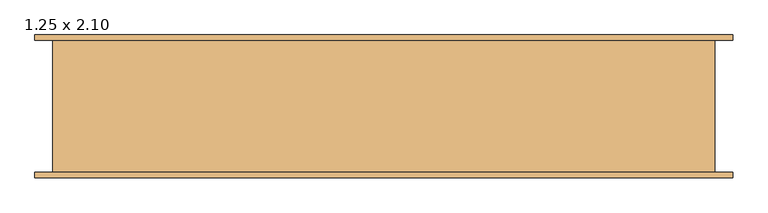
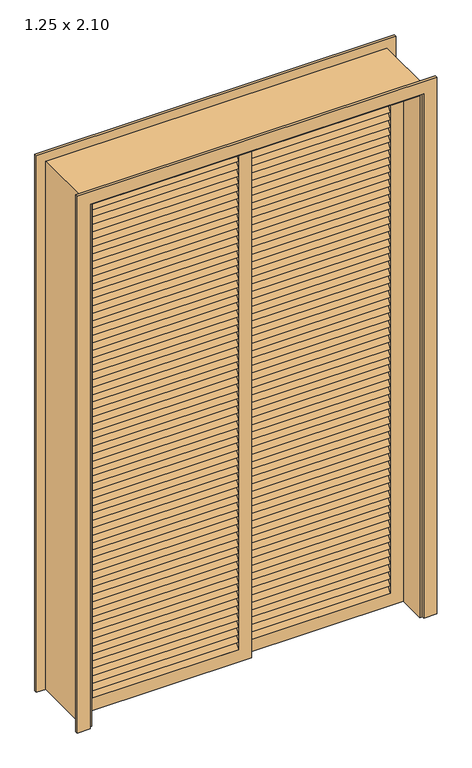
"""IFC4 building model written with IfcOpenShell, lengths in millimetres: door geometry, .CC_ND 300_PORTA DE CORRER_3 FOLHAS_VENEZIANA_VIDRO_COM EXTENSÃO : 1.25 x 2.10."""

from ifc_helpers import new_model, si_unit, frame, origin, place, context, project, spatial, polyline, outline, extrude, source, transform, mapped, element, save


def door_1_25_x_2_10_052434fb(model_context):
    return source(origin(), model_context, "Body", "SweptSolid", [
        extrude(outline(polyline([(575.0, 26.0), (20.0, 26.0), (20.0, 34.0), (575.0, 34.0), (575.0, 26.0)])), frame((0.0, 0.0, 50.0), z_axis=(0.0, 0.0, 1.0), x_axis=(1.0, 0.0, 0.0)), (0.0, 0.0, 1.0), 2000.0),
        extrude(outline(polyline([(2100.0, 625.0), (2100.0, -30.0), (0.0, -30.0), (0.0, 625.0), (2100.0, 625.0)]), holes=[polyline([(2050.0, 575.0), (50.0, 575.0), (50.0, 20.0), (2050.0, 20.0), (2050.0, 575.0)])]), frame((0.0, 15.0, 0.0), z_axis=(0.0, 1.0, 0.0), x_axis=(0.0, 0.0, 1.0)), (0.0, 0.0, 1.0), 30.0),
        extrude(outline(polyline([(-40.0, 1985.2272727), (-45.0, 1985.2272727), (-20.0, 2020.2272727), (-15.0, 2020.2272727), (-40.0, 1985.2272727)])), frame((-575.0, 0.0, 0.0), z_axis=(1.0, 0.0, 0.0), x_axis=(0.0, 1.0, 0.0)), (0.0, 0.0, 1.0), 555.0),
        extrude(outline(polyline([(-40.0, 1955.4545455), (-45.0, 1955.4545455), (-20.0, 1990.4545455), (-15.0, 1990.4545455), (-40.0, 1955.4545455)])), frame((-575.0, 0.0, 0.0), z_axis=(1.0, 0.0, 0.0), x_axis=(0.0, 1.0, 0.0)), (0.0, 0.0, 1.0), 555.0),
        extrude(outline(polyline([(-40.0, 1925.6818182), (-45.0, 1925.6818182), (-20.0, 1960.6818182), (-15.0, 1960.6818182), (-40.0, 1925.6818182)])), frame((-575.0, 0.0, 0.0), z_axis=(1.0, 0.0, 0.0), x_axis=(0.0, 1.0, 0.0)), (0.0, 0.0, 1.0), 555.0),
        extrude(outline(polyline([(-40.0, 1895.9090909), (-45.0, 1895.9090909), (-20.0, 1930.9090909), (-15.0, 1930.9090909), (-40.0, 1895.9090909)])), frame((-575.0, 0.0, 0.0), z_axis=(1.0, 0.0, 0.0), x_axis=(0.0, 1.0, 0.0)), (0.0, 0.0, 1.0), 555.0),
        extrude(outline(polyline([(-40.0, 1866.1363636), (-45.0, 1866.1363636), (-20.0, 1901.1363636), (-15.0, 1901.1363636), (-40.0, 1866.1363636)])), frame((-575.0, 0.0, 0.0), z_axis=(1.0, 0.0, 0.0), x_axis=(0.0, 1.0, 0.0)), (0.0, 0.0, 1.0), 555.0),
        extrude(outline(polyline([(-40.0, 1836.3636364), (-45.0, 1836.3636364), (-20.0, 1871.3636364), (-15.0, 1871.3636364), (-40.0, 1836.3636364)])), frame((-575.0, 0.0, 0.0), z_axis=(1.0, 0.0, 0.0), x_axis=(0.0, 1.0, 0.0)), (0.0, 0.0, 1.0), 555.0),
        extrude(outline(polyline([(-40.0, 1806.5909091), (-45.0, 1806.5909091), (-20.0, 1841.5909091), (-15.0, 1841.5909091), (-40.0, 1806.5909091)])), frame((-575.0, 0.0, 0.0), z_axis=(1.0, 0.0, 0.0), x_axis=(0.0, 1.0, 0.0)), (0.0, 0.0, 1.0), 555.0),
        extrude(outline(polyline([(-40.0, 1776.8181818), (-45.0, 1776.8181818), (-20.0, 1811.8181818), (-15.0, 1811.8181818), (-40.0, 1776.8181818)])), frame((-575.0, 0.0, 0.0), z_axis=(1.0, 0.0, 0.0), x_axis=(0.0, 1.0, 0.0)), (0.0, 0.0, 1.0), 555.0),
        extrude(outline(polyline([(-40.0, 1747.0454545), (-45.0, 1747.0454545), (-20.0, 1782.0454545), (-15.0, 1782.0454545), (-40.0, 1747.0454545)])), frame((-575.0, 0.0, 0.0), z_axis=(1.0, 0.0, 0.0), x_axis=(0.0, 1.0, 0.0)), (0.0, 0.0, 1.0), 555.0),
        extrude(outline(polyline([(-40.0, 1717.2727273), (-45.0, 1717.2727273), (-20.0, 1752.2727273), (-15.0, 1752.2727273), (-40.0, 1717.2727273)])), frame((-575.0, 0.0, 0.0), z_axis=(1.0, 0.0, 0.0), x_axis=(0.0, 1.0, 0.0)), (0.0, 0.0, 1.0), 555.0),
        extrude(outline(polyline([(-40.0, 1687.5), (-45.0, 1687.5), (-20.0, 1722.5), (-15.0, 1722.5), (-40.0, 1687.5)])), frame((-575.0, 0.0, 0.0), z_axis=(1.0, 0.0, 0.0), x_axis=(0.0, 1.0, 0.0)), (0.0, 0.0, 1.0), 555.0),
        extrude(outline(polyline([(-40.0, 1657.7272727), (-45.0, 1657.7272727), (-20.0, 1692.7272727), (-15.0, 1692.7272727), (-40.0, 1657.7272727)])), frame((-575.0, 0.0, 0.0), z_axis=(1.0, 0.0, 0.0), x_axis=(0.0, 1.0, 0.0)), (0.0, 0.0, 1.0), 555.0),
        extrude(outline(polyline([(-40.0, 1627.9545455), (-45.0, 1627.9545455), (-20.0, 1662.9545455), (-15.0, 1662.9545455), (-40.0, 1627.9545455)])), frame((-575.0, 0.0, 0.0), z_axis=(1.0, 0.0, 0.0), x_axis=(0.0, 1.0, 0.0)), (0.0, 0.0, 1.0), 555.0),
        extrude(outline(polyline([(-40.0, 1598.1818182), (-45.0, 1598.1818182), (-20.0, 1633.1818182), (-15.0, 1633.1818182), (-40.0, 1598.1818182)])), frame((-575.0, 0.0, 0.0), z_axis=(1.0, 0.0, 0.0), x_axis=(0.0, 1.0, 0.0)), (0.0, 0.0, 1.0), 555.0),
        extrude(outline(polyline([(-40.0, 1568.4090909), (-45.0, 1568.4090909), (-20.0, 1603.4090909), (-15.0, 1603.4090909), (-40.0, 1568.4090909)])), frame((-575.0, 0.0, 0.0), z_axis=(1.0, 0.0, 0.0), x_axis=(0.0, 1.0, 0.0)), (0.0, 0.0, 1.0), 555.0),
        extrude(outline(polyline([(-40.0, 1538.6363636), (-45.0, 1538.6363636), (-20.0, 1573.6363636), (-15.0, 1573.6363636), (-40.0, 1538.6363636)])), frame((-575.0, 0.0, 0.0), z_axis=(1.0, 0.0, 0.0), x_axis=(0.0, 1.0, 0.0)), (0.0, 0.0, 1.0), 555.0),
        extrude(outline(polyline([(-40.0, 1508.8636364), (-45.0, 1508.8636364), (-20.0, 1543.8636364), (-15.0, 1543.8636364), (-40.0, 1508.8636364)])), frame((-575.0, 0.0, 0.0), z_axis=(1.0, 0.0, 0.0), x_axis=(0.0, 1.0, 0.0)), (0.0, 0.0, 1.0), 555.0),
        extrude(outline(polyline([(-40.0, 1479.0909091), (-45.0, 1479.0909091), (-20.0, 1514.0909091), (-15.0, 1514.0909091), (-40.0, 1479.0909091)])), frame((-575.0, 0.0, 0.0), z_axis=(1.0, 0.0, 0.0), x_axis=(0.0, 1.0, 0.0)), (0.0, 0.0, 1.0), 555.0),
        extrude(outline(polyline([(-40.0, 1449.3181818), (-45.0, 1449.3181818), (-20.0, 1484.3181818), (-15.0, 1484.3181818), (-40.0, 1449.3181818)])), frame((-575.0, 0.0, 0.0), z_axis=(1.0, 0.0, 0.0), x_axis=(0.0, 1.0, 0.0)), (0.0, 0.0, 1.0), 555.0),
        extrude(outline(polyline([(-40.0, 1419.5454545), (-45.0, 1419.5454545), (-20.0, 1454.5454545), (-15.0, 1454.5454545), (-40.0, 1419.5454545)])), frame((-575.0, 0.0, 0.0), z_axis=(1.0, 0.0, 0.0), x_axis=(0.0, 1.0, 0.0)), (0.0, 0.0, 1.0), 555.0),
        extrude(outline(polyline([(-40.0, 1389.7727273), (-45.0, 1389.7727273), (-20.0, 1424.7727273), (-15.0, 1424.7727273), (-40.0, 1389.7727273)])), frame((-575.0, 0.0, 0.0), z_axis=(1.0, 0.0, 0.0), x_axis=(0.0, 1.0, 0.0)), (0.0, 0.0, 1.0), 555.0),
        extrude(outline(polyline([(-40.0, 1360.0), (-45.0, 1360.0), (-20.0, 1395.0), (-15.0, 1395.0), (-40.0, 1360.0)])), frame((-575.0, 0.0, 0.0), z_axis=(1.0, 0.0, 0.0), x_axis=(0.0, 1.0, 0.0)), (0.0, 0.0, 1.0), 555.0),
        extrude(outline(polyline([(-40.0, 1330.2272727), (-45.0, 1330.2272727), (-20.0, 1365.2272727), (-15.0, 1365.2272727), (-40.0, 1330.2272727)])), frame((-575.0, 0.0, 0.0), z_axis=(1.0, 0.0, 0.0), x_axis=(0.0, 1.0, 0.0)), (0.0, 0.0, 1.0), 555.0),
        extrude(outline(polyline([(-40.0, 1300.4545455), (-45.0, 1300.4545455), (-20.0, 1335.4545455), (-15.0, 1335.4545455), (-40.0, 1300.4545455)])), frame((-575.0, 0.0, 0.0), z_axis=(1.0, 0.0, 0.0), x_axis=(0.0, 1.0, 0.0)), (0.0, 0.0, 1.0), 555.0),
        extrude(outline(polyline([(-40.0, 1270.6818182), (-45.0, 1270.6818182), (-20.0, 1305.6818182), (-15.0, 1305.6818182), (-40.0, 1270.6818182)])), frame((-575.0, 0.0, 0.0), z_axis=(1.0, 0.0, 0.0), x_axis=(0.0, 1.0, 0.0)), (0.0, 0.0, 1.0), 555.0),
        extrude(outline(polyline([(-40.0, 1240.9090909), (-45.0, 1240.9090909), (-20.0, 1275.9090909), (-15.0, 1275.9090909), (-40.0, 1240.9090909)])), frame((-575.0, 0.0, 0.0), z_axis=(1.0, 0.0, 0.0), x_axis=(0.0, 1.0, 0.0)), (0.0, 0.0, 1.0), 555.0),
        extrude(outline(polyline([(-40.0, 1211.1363636), (-45.0, 1211.1363636), (-20.0, 1246.1363636), (-15.0, 1246.1363636), (-40.0, 1211.1363636)])), frame((-575.0, 0.0, 0.0), z_axis=(1.0, 0.0, 0.0), x_axis=(0.0, 1.0, 0.0)), (0.0, 0.0, 1.0), 555.0),
        extrude(outline(polyline([(-40.0, 1181.3636364), (-45.0, 1181.3636364), (-20.0, 1216.3636364), (-15.0, 1216.3636364), (-40.0, 1181.3636364)])), frame((-575.0, 0.0, 0.0), z_axis=(1.0, 0.0, 0.0), x_axis=(0.0, 1.0, 0.0)), (0.0, 0.0, 1.0), 555.0),
        extrude(outline(polyline([(-40.0, 1151.5909091), (-45.0, 1151.5909091), (-20.0, 1186.5909091), (-15.0, 1186.5909091), (-40.0, 1151.5909091)])), frame((-575.0, 0.0, 0.0), z_axis=(1.0, 0.0, 0.0), x_axis=(0.0, 1.0, 0.0)), (0.0, 0.0, 1.0), 555.0),
        extrude(outline(polyline([(-40.0, 1121.8181818), (-45.0, 1121.8181818), (-20.0, 1156.8181818), (-15.0, 1156.8181818), (-40.0, 1121.8181818)])), frame((-575.0, 0.0, 0.0), z_axis=(1.0, 0.0, 0.0), x_axis=(0.0, 1.0, 0.0)), (0.0, 0.0, 1.0), 555.0),
        extrude(outline(polyline([(-40.0, 1092.0454545), (-45.0, 1092.0454545), (-20.0, 1127.0454545), (-15.0, 1127.0454545), (-40.0, 1092.0454545)])), frame((-575.0, 0.0, 0.0), z_axis=(1.0, 0.0, 0.0), x_axis=(0.0, 1.0, 0.0)), (0.0, 0.0, 1.0), 555.0),
        extrude(outline(polyline([(-40.0, 1062.2727273), (-45.0, 1062.2727273), (-20.0, 1097.2727273), (-15.0, 1097.2727273), (-40.0, 1062.2727273)])), frame((-575.0, 0.0, 0.0), z_axis=(1.0, 0.0, 0.0), x_axis=(0.0, 1.0, 0.0)), (0.0, 0.0, 1.0), 555.0),
        extrude(outline(polyline([(-40.0, 1032.5), (-45.0, 1032.5), (-20.0, 1067.5), (-15.0, 1067.5), (-40.0, 1032.5)])), frame((-575.0, 0.0, 0.0), z_axis=(1.0, 0.0, 0.0), x_axis=(0.0, 1.0, 0.0)), (0.0, 0.0, 1.0), 555.0),
        extrude(outline(polyline([(-40.0, 1002.7272727), (-45.0, 1002.7272727), (-20.0, 1037.7272727), (-15.0, 1037.7272727), (-40.0, 1002.7272727)])), frame((-575.0, 0.0, 0.0), z_axis=(1.0, 0.0, 0.0), x_axis=(0.0, 1.0, 0.0)), (0.0, 0.0, 1.0), 555.0),
        extrude(outline(polyline([(-40.0, 972.9545455), (-45.0, 972.9545455), (-20.0, 1007.9545455), (-15.0, 1007.9545455), (-40.0, 972.9545455)])), frame((-575.0, 0.0, 0.0), z_axis=(1.0, 0.0, 0.0), x_axis=(0.0, 1.0, 0.0)), (0.0, 0.0, 1.0), 555.0),
        extrude(outline(polyline([(-40.0, 943.1818182), (-45.0, 943.1818182), (-20.0, 978.1818182), (-15.0, 978.1818182), (-40.0, 943.1818182)])), frame((-575.0, 0.0, 0.0), z_axis=(1.0, 0.0, 0.0), x_axis=(0.0, 1.0, 0.0)), (0.0, 0.0, 1.0), 555.0),
        extrude(outline(polyline([(-40.0, 913.4090909), (-45.0, 913.4090909), (-20.0, 948.4090909), (-15.0, 948.4090909), (-40.0, 913.4090909)])), frame((-575.0, 0.0, 0.0), z_axis=(1.0, 0.0, 0.0), x_axis=(0.0, 1.0, 0.0)), (0.0, 0.0, 1.0), 555.0),
        extrude(outline(polyline([(-40.0, 883.6363636), (-45.0, 883.6363636), (-20.0, 918.6363636), (-15.0, 918.6363636), (-40.0, 883.6363636)])), frame((-575.0, 0.0, 0.0), z_axis=(1.0, 0.0, 0.0), x_axis=(0.0, 1.0, 0.0)), (0.0, 0.0, 1.0), 555.0),
        extrude(outline(polyline([(-40.0, 853.8636364), (-45.0, 853.8636364), (-20.0, 888.8636364), (-15.0, 888.8636364), (-40.0, 853.8636364)])), frame((-575.0, 0.0, 0.0), z_axis=(1.0, 0.0, 0.0), x_axis=(0.0, 1.0, 0.0)), (0.0, 0.0, 1.0), 555.0),
        extrude(outline(polyline([(-40.0, 824.0909091), (-45.0, 824.0909091), (-20.0, 859.0909091), (-15.0, 859.0909091), (-40.0, 824.0909091)])), frame((-575.0, 0.0, 0.0), z_axis=(1.0, 0.0, 0.0), x_axis=(0.0, 1.0, 0.0)), (0.0, 0.0, 1.0), 555.0),
        extrude(outline(polyline([(-40.0, 794.3181818), (-45.0, 794.3181818), (-20.0, 829.3181818), (-15.0, 829.3181818), (-40.0, 794.3181818)])), frame((-575.0, 0.0, 0.0), z_axis=(1.0, 0.0, 0.0), x_axis=(0.0, 1.0, 0.0)), (0.0, 0.0, 1.0), 555.0),
        extrude(outline(polyline([(-40.0, 764.5454545), (-45.0, 764.5454545), (-20.0, 799.5454545), (-15.0, 799.5454545), (-40.0, 764.5454545)])), frame((-575.0, 0.0, 0.0), z_axis=(1.0, 0.0, 0.0), x_axis=(0.0, 1.0, 0.0)), (0.0, 0.0, 1.0), 555.0),
        extrude(outline(polyline([(-40.0, 734.7727273), (-45.0, 734.7727273), (-20.0, 769.7727273), (-15.0, 769.7727273), (-40.0, 734.7727273)])), frame((-575.0, 0.0, 0.0), z_axis=(1.0, 0.0, 0.0), x_axis=(0.0, 1.0, 0.0)), (0.0, 0.0, 1.0), 555.0),
        extrude(outline(polyline([(-40.0, 705.0), (-45.0, 705.0), (-20.0, 740.0), (-15.0, 740.0), (-40.0, 705.0)])), frame((-575.0, 0.0, 0.0), z_axis=(1.0, 0.0, 0.0), x_axis=(0.0, 1.0, 0.0)), (0.0, 0.0, 1.0), 555.0),
        extrude(outline(polyline([(-40.0, 675.2272727), (-45.0, 675.2272727), (-20.0, 710.2272727), (-15.0, 710.2272727), (-40.0, 675.2272727)])), frame((-575.0, 0.0, 0.0), z_axis=(1.0, 0.0, 0.0), x_axis=(0.0, 1.0, 0.0)), (0.0, 0.0, 1.0), 555.0),
        extrude(outline(polyline([(-40.0, 645.4545455), (-45.0, 645.4545455), (-20.0, 680.4545455), (-15.0, 680.4545455), (-40.0, 645.4545455)])), frame((-575.0, 0.0, 0.0), z_axis=(1.0, 0.0, 0.0), x_axis=(0.0, 1.0, 0.0)), (0.0, 0.0, 1.0), 555.0),
        extrude(outline(polyline([(-40.0, 615.6818182), (-45.0, 615.6818182), (-20.0, 650.6818182), (-15.0, 650.6818182), (-40.0, 615.6818182)])), frame((-575.0, 0.0, 0.0), z_axis=(1.0, 0.0, 0.0), x_axis=(0.0, 1.0, 0.0)), (0.0, 0.0, 1.0), 555.0),
        extrude(outline(polyline([(-40.0, 585.9090909), (-45.0, 585.9090909), (-20.0, 620.9090909), (-15.0, 620.9090909), (-40.0, 585.9090909)])), frame((-575.0, 0.0, 0.0), z_axis=(1.0, 0.0, 0.0), x_axis=(0.0, 1.0, 0.0)), (0.0, 0.0, 1.0), 555.0),
        extrude(outline(polyline([(-40.0, 556.1363636), (-45.0, 556.1363636), (-20.0, 591.1363636), (-15.0, 591.1363636), (-40.0, 556.1363636)])), frame((-575.0, 0.0, 0.0), z_axis=(1.0, 0.0, 0.0), x_axis=(0.0, 1.0, 0.0)), (0.0, 0.0, 1.0), 555.0),
        extrude(outline(polyline([(-40.0, 526.3636364), (-45.0, 526.3636364), (-20.0, 561.3636364), (-15.0, 561.3636364), (-40.0, 526.3636364)])), frame((-575.0, 0.0, 0.0), z_axis=(1.0, 0.0, 0.0), x_axis=(0.0, 1.0, 0.0)), (0.0, 0.0, 1.0), 555.0),
        extrude(outline(polyline([(-40.0, 496.5909091), (-45.0, 496.5909091), (-20.0, 531.5909091), (-15.0, 531.5909091), (-40.0, 496.5909091)])), frame((-575.0, 0.0, 0.0), z_axis=(1.0, 0.0, 0.0), x_axis=(0.0, 1.0, 0.0)), (0.0, 0.0, 1.0), 555.0),
        extrude(outline(polyline([(-40.0, 466.8181818), (-45.0, 466.8181818), (-20.0, 501.8181818), (-15.0, 501.8181818), (-40.0, 466.8181818)])), frame((-575.0, 0.0, 0.0), z_axis=(1.0, 0.0, 0.0), x_axis=(0.0, 1.0, 0.0)), (0.0, 0.0, 1.0), 555.0),
        extrude(outline(polyline([(-40.0, 437.0454545), (-45.0, 437.0454545), (-20.0, 472.0454545), (-15.0, 472.0454545), (-40.0, 437.0454545)])), frame((-575.0, 0.0, 0.0), z_axis=(1.0, 0.0, 0.0), x_axis=(0.0, 1.0, 0.0)), (0.0, 0.0, 1.0), 555.0),
        extrude(outline(polyline([(-40.0, 407.2727273), (-45.0, 407.2727273), (-20.0, 442.2727273), (-15.0, 442.2727273), (-40.0, 407.2727273)])), frame((-575.0, 0.0, 0.0), z_axis=(1.0, 0.0, 0.0), x_axis=(0.0, 1.0, 0.0)), (0.0, 0.0, 1.0), 555.0),
        extrude(outline(polyline([(-40.0, 377.5), (-45.0, 377.5), (-20.0, 412.5), (-15.0, 412.5), (-40.0, 377.5)])), frame((-575.0, 0.0, 0.0), z_axis=(1.0, 0.0, 0.0), x_axis=(0.0, 1.0, 0.0)), (0.0, 0.0, 1.0), 555.0),
        extrude(outline(polyline([(-40.0, 347.7272727), (-45.0, 347.7272727), (-20.0, 382.7272727), (-15.0, 382.7272727), (-40.0, 347.7272727)])), frame((-575.0, 0.0, 0.0), z_axis=(1.0, 0.0, 0.0), x_axis=(0.0, 1.0, 0.0)), (0.0, 0.0, 1.0), 555.0),
        extrude(outline(polyline([(-40.0, 317.9545455), (-45.0, 317.9545455), (-20.0, 352.9545455), (-15.0, 352.9545455), (-40.0, 317.9545455)])), frame((-575.0, 0.0, 0.0), z_axis=(1.0, 0.0, 0.0), x_axis=(0.0, 1.0, 0.0)), (0.0, 0.0, 1.0), 555.0),
        extrude(outline(polyline([(-40.0, 288.1818182), (-45.0, 288.1818182), (-20.0, 323.1818182), (-15.0, 323.1818182), (-40.0, 288.1818182)])), frame((-575.0, 0.0, 0.0), z_axis=(1.0, 0.0, 0.0), x_axis=(0.0, 1.0, 0.0)), (0.0, 0.0, 1.0), 555.0),
        extrude(outline(polyline([(-40.0, 258.4090909), (-45.0, 258.4090909), (-20.0, 293.4090909), (-15.0, 293.4090909), (-40.0, 258.4090909)])), frame((-575.0, 0.0, 0.0), z_axis=(1.0, 0.0, 0.0), x_axis=(0.0, 1.0, 0.0)), (0.0, 0.0, 1.0), 555.0),
        extrude(outline(polyline([(-40.0, 228.6363636), (-45.0, 228.6363636), (-20.0, 263.6363636), (-15.0, 263.6363636), (-40.0, 228.6363636)])), frame((-575.0, 0.0, 0.0), z_axis=(1.0, 0.0, 0.0), x_axis=(0.0, 1.0, 0.0)), (0.0, 0.0, 1.0), 555.0),
        extrude(outline(polyline([(-40.0, 198.8636364), (-45.0, 198.8636364), (-20.0, 233.8636364), (-15.0, 233.8636364), (-40.0, 198.8636364)])), frame((-575.0, 0.0, 0.0), z_axis=(1.0, 0.0, 0.0), x_axis=(0.0, 1.0, 0.0)), (0.0, 0.0, 1.0), 555.0),
        extrude(outline(polyline([(-40.0, 169.0909091), (-45.0, 169.0909091), (-20.0, 204.0909091), (-15.0, 204.0909091), (-40.0, 169.0909091)])), frame((-575.0, 0.0, 0.0), z_axis=(1.0, 0.0, 0.0), x_axis=(0.0, 1.0, 0.0)), (0.0, 0.0, 1.0), 555.0),
        extrude(outline(polyline([(-40.0, 139.3181818), (-45.0, 139.3181818), (-20.0, 174.3181818), (-15.0, 174.3181818), (-40.0, 139.3181818)])), frame((-575.0, 0.0, 0.0), z_axis=(1.0, 0.0, 0.0), x_axis=(0.0, 1.0, 0.0)), (0.0, 0.0, 1.0), 555.0),
        extrude(outline(polyline([(-40.0, 109.5454545), (-45.0, 109.5454545), (-20.0, 144.5454545), (-15.0, 144.5454545), (-40.0, 109.5454545)])), frame((-575.0, 0.0, 0.0), z_axis=(1.0, 0.0, 0.0), x_axis=(0.0, 1.0, 0.0)), (0.0, 0.0, 1.0), 555.0),
        extrude(outline(polyline([(-40.0, 79.7727273), (-45.0, 79.7727273), (-20.0, 114.7727273), (-15.0, 114.7727273), (-40.0, 79.7727273)])), frame((-575.0, 0.0, 0.0), z_axis=(1.0, 0.0, 0.0), x_axis=(0.0, 1.0, 0.0)), (0.0, 0.0, 1.0), 555.0),
        extrude(outline(polyline([(-40.0, 2015.0), (-45.0, 2015.0), (-20.0, 2050.0), (-15.0, 2050.0), (-40.0, 2015.0)])), frame((-575.0, 0.0, 0.0), z_axis=(1.0, 0.0, 0.0), x_axis=(0.0, 1.0, 0.0)), (0.0, 0.0, 1.0), 555.0),
        extrude(outline(polyline([(-40.0, 50.0), (-45.0, 50.0), (-20.0, 85.0), (-15.0, 85.0), (-40.0, 50.0)])), frame((-575.0, 0.0, 0.0), z_axis=(1.0, 0.0, 0.0), x_axis=(0.0, 1.0, 0.0)), (0.0, 0.0, 1.0), 555.0),
        extrude(outline(polyline([(2100.0, 30.0), (2100.0, -625.0), (0.0, -625.0), (0.0, 30.0), (2100.0, 30.0)]), holes=[polyline([(2050.0, -20.0), (50.0, -20.0), (50.0, -575.0), (2050.0, -575.0), (2050.0, -20.0)])]), frame((0.0, -45.0, 0.0), z_axis=(0.0, 1.0, 0.0), x_axis=(0.0, 0.0, 1.0)), (0.0, 0.0, 1.0), 30.0),
        extrude(outline(polyline([(-10.0, 1985.2272727), (-15.0, 1985.2272727), (10.0, 2020.2272727), (15.0, 2020.2272727), (-10.0, 1985.2272727)])), frame((20.0, 0.0, 0.0), z_axis=(1.0, 0.0, 0.0), x_axis=(0.0, 1.0, 0.0)), (0.0, 0.0, 1.0), 555.0),
        extrude(outline(polyline([(-10.0, 1955.4545455), (-15.0, 1955.4545455), (10.0, 1990.4545455), (15.0, 1990.4545455), (-10.0, 1955.4545455)])), frame((20.0, 0.0, 0.0), z_axis=(1.0, 0.0, 0.0), x_axis=(0.0, 1.0, 0.0)), (0.0, 0.0, 1.0), 555.0),
        extrude(outline(polyline([(-10.0, 1925.6818182), (-15.0, 1925.6818182), (10.0, 1960.6818182), (15.0, 1960.6818182), (-10.0, 1925.6818182)])), frame((20.0, 0.0, 0.0), z_axis=(1.0, 0.0, 0.0), x_axis=(0.0, 1.0, 0.0)), (0.0, 0.0, 1.0), 555.0),
        extrude(outline(polyline([(-10.0, 1895.9090909), (-15.0, 1895.9090909), (10.0, 1930.9090909), (15.0, 1930.9090909), (-10.0, 1895.9090909)])), frame((20.0, 0.0, 0.0), z_axis=(1.0, 0.0, 0.0), x_axis=(0.0, 1.0, 0.0)), (0.0, 0.0, 1.0), 555.0),
        extrude(outline(polyline([(-10.0, 1866.1363636), (-15.0, 1866.1363636), (10.0, 1901.1363636), (15.0, 1901.1363636), (-10.0, 1866.1363636)])), frame((20.0, 0.0, 0.0), z_axis=(1.0, 0.0, 0.0), x_axis=(0.0, 1.0, 0.0)), (0.0, 0.0, 1.0), 555.0),
        extrude(outline(polyline([(-10.0, 1836.3636364), (-15.0, 1836.3636364), (10.0, 1871.3636364), (15.0, 1871.3636364), (-10.0, 1836.3636364)])), frame((20.0, 0.0, 0.0), z_axis=(1.0, 0.0, 0.0), x_axis=(0.0, 1.0, 0.0)), (0.0, 0.0, 1.0), 555.0),
        extrude(outline(polyline([(-10.0, 1806.5909091), (-15.0, 1806.5909091), (10.0, 1841.5909091), (15.0, 1841.5909091), (-10.0, 1806.5909091)])), frame((20.0, 0.0, 0.0), z_axis=(1.0, 0.0, 0.0), x_axis=(0.0, 1.0, 0.0)), (0.0, 0.0, 1.0), 555.0),
        extrude(outline(polyline([(-10.0, 1776.8181818), (-15.0, 1776.8181818), (10.0, 1811.8181818), (15.0, 1811.8181818), (-10.0, 1776.8181818)])), frame((20.0, 0.0, 0.0), z_axis=(1.0, 0.0, 0.0), x_axis=(0.0, 1.0, 0.0)), (0.0, 0.0, 1.0), 555.0),
        extrude(outline(polyline([(-10.0, 1747.0454545), (-15.0, 1747.0454545), (10.0, 1782.0454545), (15.0, 1782.0454545), (-10.0, 1747.0454545)])), frame((20.0, 0.0, 0.0), z_axis=(1.0, 0.0, 0.0), x_axis=(0.0, 1.0, 0.0)), (0.0, 0.0, 1.0), 555.0),
        extrude(outline(polyline([(-10.0, 1717.2727273), (-15.0, 1717.2727273), (10.0, 1752.2727273), (15.0, 1752.2727273), (-10.0, 1717.2727273)])), frame((20.0, 0.0, 0.0), z_axis=(1.0, 0.0, 0.0), x_axis=(0.0, 1.0, 0.0)), (0.0, 0.0, 1.0), 555.0),
        extrude(outline(polyline([(-10.0, 1687.5), (-15.0, 1687.5), (10.0, 1722.5), (15.0, 1722.5), (-10.0, 1687.5)])), frame((20.0, 0.0, 0.0), z_axis=(1.0, 0.0, 0.0), x_axis=(0.0, 1.0, 0.0)), (0.0, 0.0, 1.0), 555.0),
        extrude(outline(polyline([(-10.0, 1657.7272727), (-15.0, 1657.7272727), (10.0, 1692.7272727), (15.0, 1692.7272727), (-10.0, 1657.7272727)])), frame((20.0, 0.0, 0.0), z_axis=(1.0, 0.0, 0.0), x_axis=(0.0, 1.0, 0.0)), (0.0, 0.0, 1.0), 555.0),
        extrude(outline(polyline([(-10.0, 1627.9545455), (-15.0, 1627.9545455), (10.0, 1662.9545455), (15.0, 1662.9545455), (-10.0, 1627.9545455)])), frame((20.0, 0.0, 0.0), z_axis=(1.0, 0.0, 0.0), x_axis=(0.0, 1.0, 0.0)), (0.0, 0.0, 1.0), 555.0),
        extrude(outline(polyline([(-10.0, 1598.1818182), (-15.0, 1598.1818182), (10.0, 1633.1818182), (15.0, 1633.1818182), (-10.0, 1598.1818182)])), frame((20.0, 0.0, 0.0), z_axis=(1.0, 0.0, 0.0), x_axis=(0.0, 1.0, 0.0)), (0.0, 0.0, 1.0), 555.0),
        extrude(outline(polyline([(-10.0, 1568.4090909), (-15.0, 1568.4090909), (10.0, 1603.4090909), (15.0, 1603.4090909), (-10.0, 1568.4090909)])), frame((20.0, 0.0, 0.0), z_axis=(1.0, 0.0, 0.0), x_axis=(0.0, 1.0, 0.0)), (0.0, 0.0, 1.0), 555.0),
        extrude(outline(polyline([(-10.0, 1538.6363636), (-15.0, 1538.6363636), (10.0, 1573.6363636), (15.0, 1573.6363636), (-10.0, 1538.6363636)])), frame((20.0, 0.0, 0.0), z_axis=(1.0, 0.0, 0.0), x_axis=(0.0, 1.0, 0.0)), (0.0, 0.0, 1.0), 555.0),
        extrude(outline(polyline([(-10.0, 1508.8636364), (-15.0, 1508.8636364), (10.0, 1543.8636364), (15.0, 1543.8636364), (-10.0, 1508.8636364)])), frame((20.0, 0.0, 0.0), z_axis=(1.0, 0.0, 0.0), x_axis=(0.0, 1.0, 0.0)), (0.0, 0.0, 1.0), 555.0),
        extrude(outline(polyline([(-10.0, 1479.0909091), (-15.0, 1479.0909091), (10.0, 1514.0909091), (15.0, 1514.0909091), (-10.0, 1479.0909091)])), frame((20.0, 0.0, 0.0), z_axis=(1.0, 0.0, 0.0), x_axis=(0.0, 1.0, 0.0)), (0.0, 0.0, 1.0), 555.0),
        extrude(outline(polyline([(-10.0, 1449.3181818), (-15.0, 1449.3181818), (10.0, 1484.3181818), (15.0, 1484.3181818), (-10.0, 1449.3181818)])), frame((20.0, 0.0, 0.0), z_axis=(1.0, 0.0, 0.0), x_axis=(0.0, 1.0, 0.0)), (0.0, 0.0, 1.0), 555.0),
        extrude(outline(polyline([(-10.0, 1419.5454545), (-15.0, 1419.5454545), (10.0, 1454.5454545), (15.0, 1454.5454545), (-10.0, 1419.5454545)])), frame((20.0, 0.0, 0.0), z_axis=(1.0, 0.0, 0.0), x_axis=(0.0, 1.0, 0.0)), (0.0, 0.0, 1.0), 555.0),
        extrude(outline(polyline([(-10.0, 1389.7727273), (-15.0, 1389.7727273), (10.0, 1424.7727273), (15.0, 1424.7727273), (-10.0, 1389.7727273)])), frame((20.0, 0.0, 0.0), z_axis=(1.0, 0.0, 0.0), x_axis=(0.0, 1.0, 0.0)), (0.0, 0.0, 1.0), 555.0),
        extrude(outline(polyline([(-10.0, 1360.0), (-15.0, 1360.0), (10.0, 1395.0), (15.0, 1395.0), (-10.0, 1360.0)])), frame((20.0, 0.0, 0.0), z_axis=(1.0, 0.0, 0.0), x_axis=(0.0, 1.0, 0.0)), (0.0, 0.0, 1.0), 555.0),
        extrude(outline(polyline([(-10.0, 1330.2272727), (-15.0, 1330.2272727), (10.0, 1365.2272727), (15.0, 1365.2272727), (-10.0, 1330.2272727)])), frame((20.0, 0.0, 0.0), z_axis=(1.0, 0.0, 0.0), x_axis=(0.0, 1.0, 0.0)), (0.0, 0.0, 1.0), 555.0),
        extrude(outline(polyline([(-10.0, 1300.4545455), (-15.0, 1300.4545455), (10.0, 1335.4545455), (15.0, 1335.4545455), (-10.0, 1300.4545455)])), frame((20.0, 0.0, 0.0), z_axis=(1.0, 0.0, 0.0), x_axis=(0.0, 1.0, 0.0)), (0.0, 0.0, 1.0), 555.0),
        extrude(outline(polyline([(-10.0, 1270.6818182), (-15.0, 1270.6818182), (10.0, 1305.6818182), (15.0, 1305.6818182), (-10.0, 1270.6818182)])), frame((20.0, 0.0, 0.0), z_axis=(1.0, 0.0, 0.0), x_axis=(0.0, 1.0, 0.0)), (0.0, 0.0, 1.0), 555.0),
        extrude(outline(polyline([(-10.0, 1240.9090909), (-15.0, 1240.9090909), (10.0, 1275.9090909), (15.0, 1275.9090909), (-10.0, 1240.9090909)])), frame((20.0, 0.0, 0.0), z_axis=(1.0, 0.0, 0.0), x_axis=(0.0, 1.0, 0.0)), (0.0, 0.0, 1.0), 555.0),
        extrude(outline(polyline([(-10.0, 1211.1363636), (-15.0, 1211.1363636), (10.0, 1246.1363636), (15.0, 1246.1363636), (-10.0, 1211.1363636)])), frame((20.0, 0.0, 0.0), z_axis=(1.0, 0.0, 0.0), x_axis=(0.0, 1.0, 0.0)), (0.0, 0.0, 1.0), 555.0),
        extrude(outline(polyline([(-10.0, 1181.3636364), (-15.0, 1181.3636364), (10.0, 1216.3636364), (15.0, 1216.3636364), (-10.0, 1181.3636364)])), frame((20.0, 0.0, 0.0), z_axis=(1.0, 0.0, 0.0), x_axis=(0.0, 1.0, 0.0)), (0.0, 0.0, 1.0), 555.0),
        extrude(outline(polyline([(-10.0, 1151.5909091), (-15.0, 1151.5909091), (10.0, 1186.5909091), (15.0, 1186.5909091), (-10.0, 1151.5909091)])), frame((20.0, 0.0, 0.0), z_axis=(1.0, 0.0, 0.0), x_axis=(0.0, 1.0, 0.0)), (0.0, 0.0, 1.0), 555.0),
        extrude(outline(polyline([(-10.0, 1121.8181818), (-15.0, 1121.8181818), (10.0, 1156.8181818), (15.0, 1156.8181818), (-10.0, 1121.8181818)])), frame((20.0, 0.0, 0.0), z_axis=(1.0, 0.0, 0.0), x_axis=(0.0, 1.0, 0.0)), (0.0, 0.0, 1.0), 555.0),
        extrude(outline(polyline([(-10.0, 1092.0454545), (-15.0, 1092.0454545), (10.0, 1127.0454545), (15.0, 1127.0454545), (-10.0, 1092.0454545)])), frame((20.0, 0.0, 0.0), z_axis=(1.0, 0.0, 0.0), x_axis=(0.0, 1.0, 0.0)), (0.0, 0.0, 1.0), 555.0),
        extrude(outline(polyline([(-10.0, 1062.2727273), (-15.0, 1062.2727273), (10.0, 1097.2727273), (15.0, 1097.2727273), (-10.0, 1062.2727273)])), frame((20.0, 0.0, 0.0), z_axis=(1.0, 0.0, 0.0), x_axis=(0.0, 1.0, 0.0)), (0.0, 0.0, 1.0), 555.0),
        extrude(outline(polyline([(-10.0, 1032.5), (-15.0, 1032.5), (10.0, 1067.5), (15.0, 1067.5), (-10.0, 1032.5)])), frame((20.0, 0.0, 0.0), z_axis=(1.0, 0.0, 0.0), x_axis=(0.0, 1.0, 0.0)), (0.0, 0.0, 1.0), 555.0),
        extrude(outline(polyline([(-10.0, 1002.7272727), (-15.0, 1002.7272727), (10.0, 1037.7272727), (15.0, 1037.7272727), (-10.0, 1002.7272727)])), frame((20.0, 0.0, 0.0), z_axis=(1.0, 0.0, 0.0), x_axis=(0.0, 1.0, 0.0)), (0.0, 0.0, 1.0), 555.0),
        extrude(outline(polyline([(-10.0, 972.9545455), (-15.0, 972.9545455), (10.0, 1007.9545455), (15.0, 1007.9545455), (-10.0, 972.9545455)])), frame((20.0, 0.0, 0.0), z_axis=(1.0, 0.0, 0.0), x_axis=(0.0, 1.0, 0.0)), (0.0, 0.0, 1.0), 555.0),
        extrude(outline(polyline([(-10.0, 943.1818182), (-15.0, 943.1818182), (10.0, 978.1818182), (15.0, 978.1818182), (-10.0, 943.1818182)])), frame((20.0, 0.0, 0.0), z_axis=(1.0, 0.0, 0.0), x_axis=(0.0, 1.0, 0.0)), (0.0, 0.0, 1.0), 555.0),
        extrude(outline(polyline([(-10.0, 913.4090909), (-15.0, 913.4090909), (10.0, 948.4090909), (15.0, 948.4090909), (-10.0, 913.4090909)])), frame((20.0, 0.0, 0.0), z_axis=(1.0, 0.0, 0.0), x_axis=(0.0, 1.0, 0.0)), (0.0, 0.0, 1.0), 555.0),
        extrude(outline(polyline([(-10.0, 883.6363636), (-15.0, 883.6363636), (10.0, 918.6363636), (15.0, 918.6363636), (-10.0, 883.6363636)])), frame((20.0, 0.0, 0.0), z_axis=(1.0, 0.0, 0.0), x_axis=(0.0, 1.0, 0.0)), (0.0, 0.0, 1.0), 555.0),
        extrude(outline(polyline([(-10.0, 853.8636364), (-15.0, 853.8636364), (10.0, 888.8636364), (15.0, 888.8636364), (-10.0, 853.8636364)])), frame((20.0, 0.0, 0.0), z_axis=(1.0, 0.0, 0.0), x_axis=(0.0, 1.0, 0.0)), (0.0, 0.0, 1.0), 555.0),
        extrude(outline(polyline([(-10.0, 824.0909091), (-15.0, 824.0909091), (10.0, 859.0909091), (15.0, 859.0909091), (-10.0, 824.0909091)])), frame((20.0, 0.0, 0.0), z_axis=(1.0, 0.0, 0.0), x_axis=(0.0, 1.0, 0.0)), (0.0, 0.0, 1.0), 555.0),
        extrude(outline(polyline([(-10.0, 794.3181818), (-15.0, 794.3181818), (10.0, 829.3181818), (15.0, 829.3181818), (-10.0, 794.3181818)])), frame((20.0, 0.0, 0.0), z_axis=(1.0, 0.0, 0.0), x_axis=(0.0, 1.0, 0.0)), (0.0, 0.0, 1.0), 555.0),
        extrude(outline(polyline([(-10.0, 764.5454545), (-15.0, 764.5454545), (10.0, 799.5454545), (15.0, 799.5454545), (-10.0, 764.5454545)])), frame((20.0, 0.0, 0.0), z_axis=(1.0, 0.0, 0.0), x_axis=(0.0, 1.0, 0.0)), (0.0, 0.0, 1.0), 555.0),
        extrude(outline(polyline([(-10.0, 734.7727273), (-15.0, 734.7727273), (10.0, 769.7727273), (15.0, 769.7727273), (-10.0, 734.7727273)])), frame((20.0, 0.0, 0.0), z_axis=(1.0, 0.0, 0.0), x_axis=(0.0, 1.0, 0.0)), (0.0, 0.0, 1.0), 555.0),
        extrude(outline(polyline([(-10.0, 705.0), (-15.0, 705.0), (10.0, 740.0), (15.0, 740.0), (-10.0, 705.0)])), frame((20.0, 0.0, 0.0), z_axis=(1.0, 0.0, 0.0), x_axis=(0.0, 1.0, 0.0)), (0.0, 0.0, 1.0), 555.0),
        extrude(outline(polyline([(-10.0, 675.2272727), (-15.0, 675.2272727), (10.0, 710.2272727), (15.0, 710.2272727), (-10.0, 675.2272727)])), frame((20.0, 0.0, 0.0), z_axis=(1.0, 0.0, 0.0), x_axis=(0.0, 1.0, 0.0)), (0.0, 0.0, 1.0), 555.0),
        extrude(outline(polyline([(-10.0, 645.4545455), (-15.0, 645.4545455), (10.0, 680.4545455), (15.0, 680.4545455), (-10.0, 645.4545455)])), frame((20.0, 0.0, 0.0), z_axis=(1.0, 0.0, 0.0), x_axis=(0.0, 1.0, 0.0)), (0.0, 0.0, 1.0), 555.0),
        extrude(outline(polyline([(-10.0, 615.6818182), (-15.0, 615.6818182), (10.0, 650.6818182), (15.0, 650.6818182), (-10.0, 615.6818182)])), frame((20.0, 0.0, 0.0), z_axis=(1.0, 0.0, 0.0), x_axis=(0.0, 1.0, 0.0)), (0.0, 0.0, 1.0), 555.0),
        extrude(outline(polyline([(-10.0, 585.9090909), (-15.0, 585.9090909), (10.0, 620.9090909), (15.0, 620.9090909), (-10.0, 585.9090909)])), frame((20.0, 0.0, 0.0), z_axis=(1.0, 0.0, 0.0), x_axis=(0.0, 1.0, 0.0)), (0.0, 0.0, 1.0), 555.0),
        extrude(outline(polyline([(-10.0, 556.1363636), (-15.0, 556.1363636), (10.0, 591.1363636), (15.0, 591.1363636), (-10.0, 556.1363636)])), frame((20.0, 0.0, 0.0), z_axis=(1.0, 0.0, 0.0), x_axis=(0.0, 1.0, 0.0)), (0.0, 0.0, 1.0), 555.0),
        extrude(outline(polyline([(-10.0, 526.3636364), (-15.0, 526.3636364), (10.0, 561.3636364), (15.0, 561.3636364), (-10.0, 526.3636364)])), frame((20.0, 0.0, 0.0), z_axis=(1.0, 0.0, 0.0), x_axis=(0.0, 1.0, 0.0)), (0.0, 0.0, 1.0), 555.0),
        extrude(outline(polyline([(-10.0, 496.5909091), (-15.0, 496.5909091), (10.0, 531.5909091), (15.0, 531.5909091), (-10.0, 496.5909091)])), frame((20.0, 0.0, 0.0), z_axis=(1.0, 0.0, 0.0), x_axis=(0.0, 1.0, 0.0)), (0.0, 0.0, 1.0), 555.0),
        extrude(outline(polyline([(-10.0, 466.8181818), (-15.0, 466.8181818), (10.0, 501.8181818), (15.0, 501.8181818), (-10.0, 466.8181818)])), frame((20.0, 0.0, 0.0), z_axis=(1.0, 0.0, 0.0), x_axis=(0.0, 1.0, 0.0)), (0.0, 0.0, 1.0), 555.0),
        extrude(outline(polyline([(-10.0, 437.0454545), (-15.0, 437.0454545), (10.0, 472.0454545), (15.0, 472.0454545), (-10.0, 437.0454545)])), frame((20.0, 0.0, 0.0), z_axis=(1.0, 0.0, 0.0), x_axis=(0.0, 1.0, 0.0)), (0.0, 0.0, 1.0), 555.0),
        extrude(outline(polyline([(-10.0, 407.2727273), (-15.0, 407.2727273), (10.0, 442.2727273), (15.0, 442.2727273), (-10.0, 407.2727273)])), frame((20.0, 0.0, 0.0), z_axis=(1.0, 0.0, 0.0), x_axis=(0.0, 1.0, 0.0)), (0.0, 0.0, 1.0), 555.0),
        extrude(outline(polyline([(-10.0, 377.5), (-15.0, 377.5), (10.0, 412.5), (15.0, 412.5), (-10.0, 377.5)])), frame((20.0, 0.0, 0.0), z_axis=(1.0, 0.0, 0.0), x_axis=(0.0, 1.0, 0.0)), (0.0, 0.0, 1.0), 555.0),
        extrude(outline(polyline([(-10.0, 347.7272727), (-15.0, 347.7272727), (10.0, 382.7272727), (15.0, 382.7272727), (-10.0, 347.7272727)])), frame((20.0, 0.0, 0.0), z_axis=(1.0, 0.0, 0.0), x_axis=(0.0, 1.0, 0.0)), (0.0, 0.0, 1.0), 555.0),
        extrude(outline(polyline([(-10.0, 317.9545455), (-15.0, 317.9545455), (10.0, 352.9545455), (15.0, 352.9545455), (-10.0, 317.9545455)])), frame((20.0, 0.0, 0.0), z_axis=(1.0, 0.0, 0.0), x_axis=(0.0, 1.0, 0.0)), (0.0, 0.0, 1.0), 555.0),
        extrude(outline(polyline([(-10.0, 288.1818182), (-15.0, 288.1818182), (10.0, 323.1818182), (15.0, 323.1818182), (-10.0, 288.1818182)])), frame((20.0, 0.0, 0.0), z_axis=(1.0, 0.0, 0.0), x_axis=(0.0, 1.0, 0.0)), (0.0, 0.0, 1.0), 555.0),
        extrude(outline(polyline([(-10.0, 258.4090909), (-15.0, 258.4090909), (10.0, 293.4090909), (15.0, 293.4090909), (-10.0, 258.4090909)])), frame((20.0, 0.0, 0.0), z_axis=(1.0, 0.0, 0.0), x_axis=(0.0, 1.0, 0.0)), (0.0, 0.0, 1.0), 555.0),
        extrude(outline(polyline([(-10.0, 228.6363636), (-15.0, 228.6363636), (10.0, 263.6363636), (15.0, 263.6363636), (-10.0, 228.6363636)])), frame((20.0, 0.0, 0.0), z_axis=(1.0, 0.0, 0.0), x_axis=(0.0, 1.0, 0.0)), (0.0, 0.0, 1.0), 555.0),
        extrude(outline(polyline([(-10.0, 198.8636364), (-15.0, 198.8636364), (10.0, 233.8636364), (15.0, 233.8636364), (-10.0, 198.8636364)])), frame((20.0, 0.0, 0.0), z_axis=(1.0, 0.0, 0.0), x_axis=(0.0, 1.0, 0.0)), (0.0, 0.0, 1.0), 555.0),
        extrude(outline(polyline([(-10.0, 169.0909091), (-15.0, 169.0909091), (10.0, 204.0909091), (15.0, 204.0909091), (-10.0, 169.0909091)])), frame((20.0, 0.0, 0.0), z_axis=(1.0, 0.0, 0.0), x_axis=(0.0, 1.0, 0.0)), (0.0, 0.0, 1.0), 555.0),
        extrude(outline(polyline([(-10.0, 139.3181818), (-15.0, 139.3181818), (10.0, 174.3181818), (15.0, 174.3181818), (-10.0, 139.3181818)])), frame((20.0, 0.0, 0.0), z_axis=(1.0, 0.0, 0.0), x_axis=(0.0, 1.0, 0.0)), (0.0, 0.0, 1.0), 555.0),
        extrude(outline(polyline([(-10.0, 109.5454545), (-15.0, 109.5454545), (10.0, 144.5454545), (15.0, 144.5454545), (-10.0, 109.5454545)])), frame((20.0, 0.0, 0.0), z_axis=(1.0, 0.0, 0.0), x_axis=(0.0, 1.0, 0.0)), (0.0, 0.0, 1.0), 555.0),
        extrude(outline(polyline([(-10.0, 79.7727273), (-15.0, 79.7727273), (10.0, 114.7727273), (15.0, 114.7727273), (-10.0, 79.7727273)])), frame((20.0, 0.0, 0.0), z_axis=(1.0, 0.0, 0.0), x_axis=(0.0, 1.0, 0.0)), (0.0, 0.0, 1.0), 555.0),
        extrude(outline(polyline([(-10.0, 2015.0), (-15.0, 2015.0), (10.0, 2050.0), (15.0, 2050.0), (-10.0, 2015.0)])), frame((20.0, 0.0, 0.0), z_axis=(1.0, 0.0, 0.0), x_axis=(0.0, 1.0, 0.0)), (0.0, 0.0, 1.0), 555.0),
        extrude(outline(polyline([(-10.0, 50.0), (-15.0, 50.0), (10.0, 85.0), (15.0, 85.0), (-10.0, 50.0)])), frame((20.0, 0.0, 0.0), z_axis=(1.0, 0.0, 0.0), x_axis=(0.0, 1.0, 0.0)), (0.0, 0.0, 1.0), 555.0),
        extrude(outline(polyline([(2100.0, 625.0), (2100.0, -30.0), (0.0, -30.0), (0.0, 625.0), (2100.0, 625.0)]), holes=[polyline([(2050.0, 575.0), (50.0, 575.0), (50.0, 20.0), (2050.0, 20.0), (2050.0, 575.0)])]), frame((0.0, -15.0, 0.0), z_axis=(0.0, 1.0, 0.0), x_axis=(0.0, 0.0, 1.0)), (0.0, 0.0, 1.0), 30.0),
        extrude(outline(polyline([(0.0, 685.0), (2160.0, 685.0), (2160.0, -685.0), (0.0, -685.0), (0.0, -635.0), (2110.0, -635.0), (2110.0, 635.0), (0.0, 635.0), (0.0, 685.0)])), frame((0.0, -132.4, 0.0), z_axis=(0.0, 1.0, 0.0), x_axis=(0.0, 0.0, 1.0)), (0.0, 0.0, 1.0), 10.0),
        extrude(outline(polyline([(0.0, -635.0), (2110.0, -635.0), (2110.0, 635.0), (0.0, 635.0), (0.0, 685.0), (2160.0, 685.0), (2160.0, -685.0), (0.0, -685.0), (0.0, -635.0)])), frame((0.0, 137.4, 0.0), z_axis=(0.0, 1.0, 0.0), x_axis=(0.0, 0.0, 1.0)), (0.0, 0.0, 1.0), 10.0),
        extrude(outline(polyline([(0.0, -625.0), (2100.0, -625.0), (2100.0, 625.0), (0.0, 625.0), (0.0, 650.0), (2125.0, 650.0), (2125.0, -650.0), (0.0, -650.0), (0.0, -625.0)])), frame((0.0, -122.4, 0.0), z_axis=(0.0, 1.0, 0.0), x_axis=(0.0, 0.0, 1.0)), (0.0, 0.0, 1.0), 259.8),
    ])


if __name__ == "__main__":
    model = new_model("IFC4")
    model_context = context("Model", 3, world=origin())
    ifc_project = project(units=[si_unit("LENGTHUNIT", "METRE", prefix="MILLI")], contexts=[model_context])
    site = spatial("IfcSite", under=ifc_project)
    building = spatial("IfcBuilding", under=site)
    placement = place(None, origin())
    door_1_25_x_2_10_shape = door_1_25_x_2_10_052434fb(model_context)
    element("IfcDoor", 1, ObjectType=".CC_ND 300_PORTA DE CORRER_3 FOLHAS_VENEZIANA_VIDRO_COM EXTENSÃO : 1.25 x 2.10", at=placement, inside=building, context=model_context, shape_type="MappedRepresentation", body=[
        mapped(door_1_25_x_2_10_shape, transform((0.0, 0.0, 0.0), x_axis=(1.0, 0.0, 0.0), y_axis=(0.0, 1.0, 0.0), z_axis=(0.0, 0.0, 1.0))),
    ])
    save(model, "model.ifc")

# Revit data of these elements
# Type ".CC_ND 300_PORTA DE CORRER_3 FOLHAS_VENEZIANA_VIDRO_COM EXTENSÃO : 1.25 x 2.10"
#   Type Mark = "152"
#   Analytic Construction = "<Nenhum>"
#   Extensão acabamento interior [instance default] = 0.00 m
#   Extensão acabamento exterior [instance default] = 0.00 m
#   Espessura vidro = 0.008 m
#   Largura painéis vidro e veneziana = 0.03 m
#   Largura moldura = 0.05 m
#   Rough Width = 1.30 m
#   Largura painéis = 0.655 m
#   Espessura painéis vidro e veneziana = 0.03 m
#   Espessura moldura = 0.01 m
#   Espessura batente = 0.025 m
#   Rough Height = 2.125 m
#   Height = 2.10 m
#   Width = 1.25 m
#   Moldura interna [instance default] = yes
#   Moldura externa [instance default] = yes
#   Function = 1
#   Vidro = .VIDRO GENÉRICO
#   Batente = .ALUMÍNIO COM PINTURA ELETROSTÁTICA BRANCA
#   Moldura = .ALUMÍNIO COM PINTURA ELETROSTÁTICA BRANCA
#   Painéis = .ALUMÍNIO COM PINTURA ELETROSTÁTICA BRANCA
#   Thickness = 0
#   Wall Closure = (empty or 0)
# Element 1 (IfcDoor, ".CC_ND 300_PORTA DE CORRER_3 FOLHAS_VENEZIANA_VIDRO_COM EXTENSÃO : 1.25 x 2.10")
#   Materials on its faces: ".ALUMÍNIO COM PINTURA ELETROSTÁTICA BRANCA", ".VIDRO GENÉRICO"
# Materials
#   ".VIDRO GENÉRICO": class ".CC_VIDRO", colour RGB 0 128 192, transparency 0.9, Description = "Vidro comum", Cost = 0
#   ".ALUMÍNIO COM PINTURA ELETROSTÁTICA BRANCA": class "CC_METAIS", colour RGB 241 241 241, transparency 0, Cost = 0
